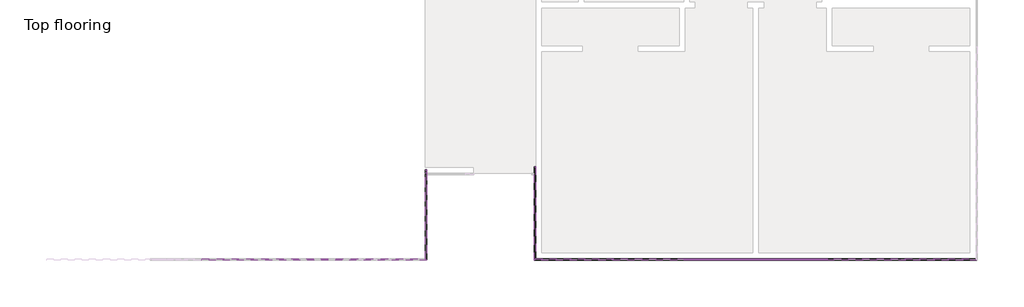
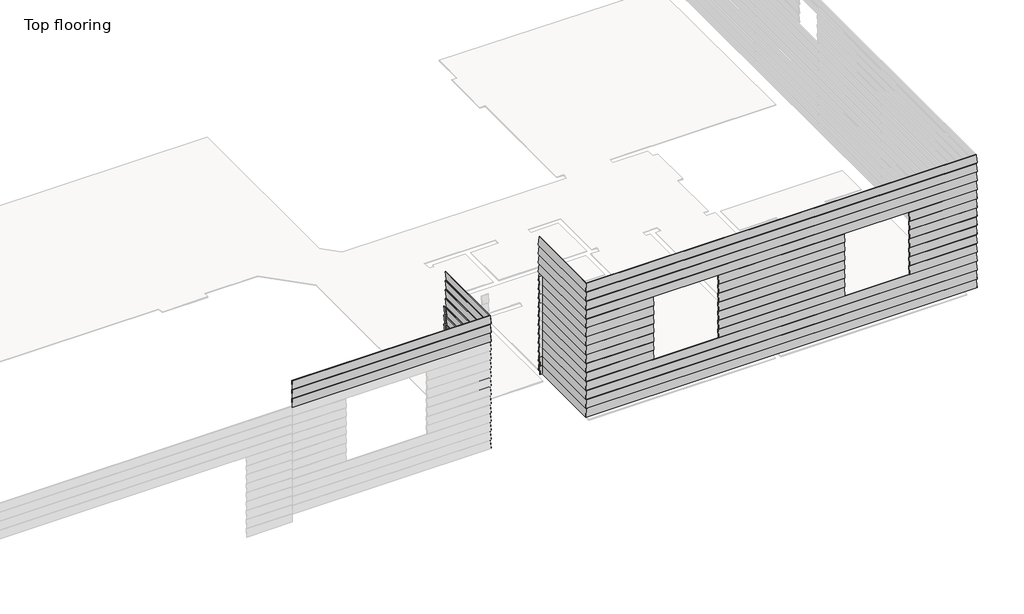
# One storey, part 2 of 5: 50 proxies.
"""IFC4 building model written with IfcOpenShell, lengths in millimetres."""

import ifcopenshell
import ifcopenshell.guid

model = None  # the IFC model being written
_history = None  # IfcOwnerHistory: only IFC2X3 demands one
_inside = {}  # id of a spatial element -> (the spatial element, [elements in it])
_under = {}  # id of a project, library or spatial element -> (it, [spatial elements below it])
_declared = {}  # id of a project -> (the project, [libraries it declares])
_typed = {}  # id of a type object -> (the type object, [elements of that type])
_made_of = {}  # id of a material, layer set ... -> (it, [elements and type objects made of it])


def new_model(schema):
    """Start an empty IFC model of exactly this schema.

    Asked for "IFC4X3", IfcOpenShell would pick the latest addendum, in which some entities
    have other attributes; the version numbers below select the first issue.
    IFC2X3 requires an IfcOwnerHistory on every rooted entity: one is made here for all.
    """
    global model, _history
    if schema == "IFC4X3":
        model = ifcopenshell.file(schema_version=(4, 3, 0, 0))
    else:
        model = ifcopenshell.file(schema=schema)
    _inside.clear()
    _under.clear()
    _declared.clear()
    _typed.clear()
    _made_of.clear()
    _history = None
    if model.schema == "IFC2X3":
        org = make("IfcOrganization", Name="unknown")
        user = make(
            "IfcPersonAndOrganization",
            ThePerson=make("IfcPerson", FamilyName="unknown"),
            TheOrganization=org,
        )
        app = make(
            "IfcApplication",
            ApplicationDeveloper=org,
            Version="unknown",
            ApplicationFullName="unknown",
            ApplicationIdentifier="unknown",
        )
        _history = make(
            "IfcOwnerHistory",
            OwningUser=user,
            OwningApplication=app,
            ChangeAction="ADDED",
            CreationDate=0,
        )
    return model


def make(cls, **values):
    """One entity of the class cls with the attributes given. An attribute that is None is left unset."""
    return model.create_entity(
        cls, **{name: value for name, value in values.items() if value is not None}
    )


def rooted(cls, **values):
    """An entity with a GlobalId (a new one), such as an element, a storey or a relation."""
    return make(cls, GlobalId=ifcopenshell.guid.new(), OwnerHistory=_history, **values)


def si_unit(unit_type, name, prefix=None):
    """IfcSIUnit, for example si_unit("LENGTHUNIT", "METRE", prefix="MILLI")."""
    return make("IfcSIUnit", UnitType=unit_type, Prefix=prefix, Name=name)


def assignment(units):
    """IfcUnitAssignment: the units of a project."""
    return None if units is None else make("IfcUnitAssignment", Units=units)


def point(xyz):
    """IfcCartesianPoint."""
    return None if xyz is None else make("IfcCartesianPoint", Coordinates=xyz)


def direction(xyz):
    """IfcDirection."""
    return None if xyz is None else make("IfcDirection", DirectionRatios=xyz)


def frame(location, z_axis=None, x_axis=None):
    """IfcAxis2Placement3D, a coordinate frame: its origin and axes. An axis left out is left unset."""
    return make(
        "IfcAxis2Placement3D",
        Location=point(location),
        Axis=direction(z_axis),
        RefDirection=direction(x_axis),
    )


def origin():
    """The frame at (0, 0, 0) with its axes left unset."""
    return frame((0.0, 0.0, 0.0))


def place(relative_to, where):
    """IfcLocalPlacement: puts the frame where relative to a parent placement (None: the world)."""
    return make(
        "IfcLocalPlacement", PlacementRelTo=relative_to, RelativePlacement=where
    )


def context(
    kind, dimensions, precision=None, world=None, true_north=None, identifier=None
):
    """IfcGeometricRepresentationContext, for example the 3D "Model" context."""
    return make(
        "IfcGeometricRepresentationContext",
        ContextIdentifier=identifier,
        ContextType=kind,
        CoordinateSpaceDimension=dimensions,
        Precision=precision,
        WorldCoordinateSystem=world,
        TrueNorth=true_north,
    )


def project(units=None, contexts=None):
    """IfcProject with its units and contexts."""
    return rooted(
        "IfcProject",
        Name="project",
        RepresentationContexts=contexts,
        UnitsInContext=assignment(units),
    )


def spatial(cls, under=None, at=None, **own):
    """A site, building, storey or space (cls), placed at a placement, below another one or the project."""
    s = rooted(cls, ObjectPlacement=at, **own)
    if under is not None:
        _under.setdefault(under.id(), (under, []))[1].append(s)
    return s


def polyline(points):
    """IfcPolyline through the points."""
    return make("IfcPolyline", Points=[point(p) for p in points])


def outline(outer, holes=None, kind="AREA"):
    """IfcArbitraryClosedProfileDef: a profile drawn as a closed curve; with holes, ...WithVoids."""
    if holes is None:
        return make("IfcArbitraryClosedProfileDef", ProfileType=kind, OuterCurve=outer)
    return make(
        "IfcArbitraryProfileDefWithVoids",
        ProfileType=kind,
        OuterCurve=outer,
        InnerCurves=holes,
    )


def extrude(swept, where, along, depth):
    """IfcExtrudedAreaSolid: the profile swept, set in the frame where, extruded along a direction by depth."""
    return make(
        "IfcExtrudedAreaSolid",
        SweptArea=swept,
        Position=where,
        ExtrudedDirection=direction(along),
        Depth=depth,
    )


def faces_of(points, faces, orient=None, outer=None):
    """IfcFace entities. A face is a list of loops; a loop is a list of indices into points, from 0.

    orient and outer hold one flag for each loop. By default every Orientation is true, the
    first loop of a face is its IfcFaceOuterBound and the others are IfcFaceBound.
    """
    made = []
    for i, loops in enumerate(faces):
        bounds = []
        for j, loop in enumerate(loops):
            is_outer = j == 0 if outer is None else outer[i][j]
            bounds.append(
                make(
                    "IfcFaceOuterBound" if is_outer else "IfcFaceBound",
                    Bound=make("IfcPolyLoop", Polygon=[points[k] for k in loop]),
                    Orientation=True if orient is None else orient[i][j],
                )
            )
        made.append(make("IfcFace", Bounds=bounds))
    return made


def faceted_brep(points, faces, orient=None, outer=None, voids=None):
    """IfcFacetedBrep: a solid bounded by flat faces; with voids (closed shells), ...WithVoids."""
    shared = [point(p) for p in points]
    hull = make("IfcClosedShell", CfsFaces=faces_of(shared, faces, orient, outer))
    if voids is None:
        return make("IfcFacetedBrep", Outer=hull)
    return make(
        "IfcFacetedBrepWithVoids",
        Outer=hull,
        Voids=[
            make(cls, CfsFaces=faces_of(shared, fs, o, b)) for cls, fs, o, b in voids
        ],
    )


def shape(context_of_items, identifier, shape_type, items):
    """IfcShapeRepresentation: the items that make up one representation, for example the "Body"."""
    return make(
        "IfcShapeRepresentation",
        ContextOfItems=context_of_items,
        RepresentationIdentifier=identifier,
        RepresentationType=shape_type,
        Items=items,
    )


def made_of(thing, what):
    """Note that an element or type object is made of a material, layer set ...; save() writes the relation."""
    if what is not None:
        _made_of.setdefault(what.id(), (what, []))[1].append(thing)
    return thing


def element(
    cls,
    number,
    at=None,
    inside=None,
    cuts=None,
    type_object=None,
    material=None,
    context=None,
    identifier="Body",
    shape_type=None,
    held_by="IfcProductDefinitionShape",
    body=None,
    shapes=None,
    **own,
):
    """One element of the class cls, such as IfcWall. Its Tag is "e" and its number.

    at: its placement. inside: the storey or other place that contains it. cuts: it is an
    opening in that element (IfcRelVoidsElement). A single representation is given by context,
    identifier, shape_type and body (its items); several are given by shapes. held_by: the class
    of the entity that holds the representations. save() writes the other relations.
    """
    e = rooted(cls, Tag="e%d" % number, ObjectPlacement=at, **own)
    if body is not None:
        shapes = [shape(context, identifier, shape_type, body)]
    if shapes is not None:
        e.Representation = make(held_by, Representations=shapes)
    if inside is not None:
        _inside.setdefault(inside.id(), (inside, []))[1].append(e)
    if cuts is not None:
        rooted(
            "IfcRelVoidsElement", RelatingBuildingElement=cuts, RelatedOpeningElement=e
        )
    if type_object is not None:
        _typed.setdefault(type_object.id(), (type_object, []))[1].append(e)
    return made_of(e, material)


def aggregate(whole, parts):
    """IfcRelAggregates: a whole, such as a stair, and the parts it consists of."""
    return rooted("IfcRelAggregates", RelatingObject=whole, RelatedObjects=parts)


def save(model, path):
    """Write the relations noted so far, then the file.

    IfcRelAggregates (storeys below a building ...), IfcRelContainedInSpatialStructure (elements
    in a storey), IfcRelDefinesByType, IfcRelAssociatesMaterial and IfcRelDeclares: one each for
    every whole, place, type object, material and project.
    """
    for whole, parts in _under.values():
        aggregate(whole, parts)
    for where, things in _inside.values():
        rooted(
            "IfcRelContainedInSpatialStructure",
            RelatedElements=things,
            RelatingStructure=where,
        )
    for kind, things in _typed.values():
        rooted("IfcRelDefinesByType", RelatedObjects=things, RelatingType=kind)
    for what, things in _made_of.values():
        rooted("IfcRelAssociatesMaterial", RelatedObjects=things, RelatingMaterial=what)
    for by, libraries in _declared.values():
        rooted("IfcRelDeclares", RelatingContext=by, RelatedDefinitions=libraries)
    model.write(path)


model = new_model("IFC4")

# Units and contexts
model_context = context("Model", 3, world=origin())
ifc_project = project(units=[si_unit("LENGTHUNIT", "METRE", prefix="MILLI")], contexts=[model_context])

# Site, building, storey
site = spatial("IfcSite", under=ifc_project)
building = spatial("IfcBuilding", under=site)
storey = spatial("IfcBuildingStorey", under=building, Name="Top flooring", Elevation=12.7)

# Proxies
placement = place(None, origin())
element("IfcBuildingElementProxy", 1, Name="Wall Sweeps", at=placement, inside=storey, context=model_context, shape_type="Brep", body=[
    faceted_brep([(-7413.8787386, -5078.007679, 179.3151454), (-7428.0541529, -5063.8322648, 338.6859634), (-7438.014829, -5053.8715886, 337.8), (-7423.8394147, -5068.0470029, 178.429182), (-7413.8787386, -3576.793764, 179.3151454), (-7423.8394147, -3576.793764, 178.429182), (-7438.014829, -3576.793764, 337.8), (-7428.0541529, -3576.793764, 338.6859634)], [[[0, 1, 2, 3]], [[4, 5, 6, 7]], [[1, 0, 4, 7]], [[2, 1, 7, 6]], [[3, 2, 6, 5]], [[0, 3, 5, 4]]]),
])
element("IfcBuildingElementProxy", 2, Name="Wall Sweeps", at=placement, inside=storey, context=model_context, shape_type="Brep", body=[
    faceted_brep([(-7413.8787386, -5078.007679, 357.1151454), (-7428.0541529, -5063.8322648, 516.4859634), (-7438.014829, -5053.8715886, 515.6), (-7423.8394147, -5068.0470029, 356.229182), (-7413.8787386, -3576.793764, 357.1151454), (-7423.8394147, -3576.793764, 356.229182), (-7438.014829, -3576.793764, 515.6), (-7428.0541529, -3576.793764, 516.4859634)], [[[0, 1, 2, 3]], [[4, 5, 6, 7]], [[1, 0, 4, 7]], [[2, 1, 7, 6]], [[3, 2, 6, 5]], [[0, 3, 5, 4]]]),
])
element("IfcBuildingElementProxy", 3, Name="Wall Sweeps", at=placement, inside=storey, context=model_context, shape_type="Brep", body=[
    faceted_brep([(-7413.8787386, -5078.007679, 534.9151454), (-7428.0541529, -5063.8322648, 694.2859634), (-7438.014829, -5053.8715886, 693.4), (-7423.8394147, -5068.0470029, 534.029182), (-7413.8787386, -3576.793764, 534.9151454), (-7423.8394147, -3576.793764, 534.029182), (-7438.014829, -3576.793764, 693.4), (-7428.0541529, -3576.793764, 694.2859634)], [[[0, 1, 2, 3]], [[4, 5, 6, 7]], [[1, 0, 4, 7]], [[2, 1, 7, 6]], [[3, 2, 6, 5]], [[0, 3, 5, 4]]]),
])
element("IfcBuildingElementProxy", 4, Name="Wall Sweeps", at=placement, inside=storey, context=model_context, shape_type="Brep", body=[
    faceted_brep([(-7413.8787386, -5078.007679, 712.7151454), (-7428.0541529, -5063.8322648, 872.0859634), (-7438.014829, -5053.8715886, 871.2), (-7423.8394147, -5068.0470029, 711.829182), (-7413.8787386, -3576.793764, 712.7151454), (-7423.8394147, -3576.793764, 711.829182), (-7438.014829, -3576.793764, 871.2), (-7428.0541529, -3576.793764, 872.0859634)], [[[0, 1, 2, 3]], [[4, 5, 6, 7]], [[1, 0, 4, 7]], [[2, 1, 7, 6]], [[3, 2, 6, 5]], [[0, 3, 5, 4]]]),
])
element("IfcBuildingElementProxy", 5, Name="Wall Sweeps", at=placement, inside=storey, context=model_context, shape_type="Brep", body=[
    faceted_brep([(-7413.8787386, -5078.007679, 890.5151454), (-7428.0541529, -5063.8322648, 1049.8859634), (-7438.014829, -5053.8715886, 1049.0), (-7423.8394147, -5068.0470029, 889.629182), (-7413.8787386, -3576.793764, 890.5151454), (-7423.8394147, -3576.793764, 889.629182), (-7438.014829, -3576.793764, 1049.0), (-7428.0541529, -3576.793764, 1049.8859634)], [[[0, 1, 2, 3]], [[4, 5, 6, 7]], [[1, 0, 4, 7]], [[2, 1, 7, 6]], [[3, 2, 6, 5]], [[0, 3, 5, 4]]]),
])
element("IfcBuildingElementProxy", 6, Name="Wall Sweeps", at=placement, inside=storey, context=model_context, shape_type="Brep", body=[
    faceted_brep([(-7413.8787386, -5078.007679, 1068.3151454), (-7428.0541529, -5063.8322648, 1227.6859634), (-7438.014829, -5053.8715886, 1226.8), (-7423.8394147, -5068.0470029, 1067.429182), (-7413.8787386, -3576.793764, 1068.3151454), (-7423.8394147, -3576.793764, 1067.429182), (-7438.014829, -3576.793764, 1226.8), (-7428.0541529, -3576.793764, 1227.6859634)], [[[0, 1, 2, 3]], [[4, 5, 6, 7]], [[1, 0, 4, 7]], [[2, 1, 7, 6]], [[3, 2, 6, 5]], [[0, 3, 5, 4]]]),
])
element("IfcBuildingElementProxy", 7, Name="Wall Sweeps", at=placement, inside=storey, context=model_context, shape_type="Brep", body=[
    faceted_brep([(-7413.8787386, -5078.007679, 1246.1151454), (-7428.0541529, -5063.8322648, 1405.4859634), (-7438.014829, -5053.8715886, 1404.6), (-7423.8394147, -5068.0470029, 1245.229182), (-7413.8787386, -3576.793764, 1246.1151454), (-7423.8394147, -3576.793764, 1245.229182), (-7438.014829, -3576.793764, 1404.6), (-7428.0541529, -3576.793764, 1405.4859634)], [[[0, 1, 2, 3]], [[4, 5, 6, 7]], [[1, 0, 4, 7]], [[2, 1, 7, 6]], [[3, 2, 6, 5]], [[0, 3, 5, 4]]]),
])
element("IfcBuildingElementProxy", 8, Name="Wall Sweeps", at=placement, inside=storey, context=model_context, shape_type="Brep", body=[
    faceted_brep([(-7413.8787386, -5078.007679, 1423.9151454), (-7428.0541529, -5063.8322648, 1583.2859634), (-7438.014829, -5053.8715886, 1582.4), (-7423.8394147, -5068.0470029, 1423.029182), (-7413.8787386, -3576.793764, 1423.9151454), (-7423.8394147, -3576.793764, 1423.029182), (-7438.014829, -3576.793764, 1582.4), (-7428.0541529, -3576.793764, 1583.2859634)], [[[0, 1, 2, 3]], [[4, 5, 6, 7]], [[1, 0, 4, 7]], [[2, 1, 7, 6]], [[3, 2, 6, 5]], [[0, 3, 5, 4]]]),
])
element("IfcBuildingElementProxy", 9, Name="Wall Sweeps", at=placement, inside=storey, context=model_context, shape_type="Brep", body=[
    faceted_brep([(-7413.8787386, -5078.007679, 1601.7151454), (-7428.0541529, -5063.8322648, 1761.0859634), (-7438.014829, -5053.8715886, 1760.2), (-7423.8394147, -5068.0470029, 1600.829182), (-7413.8787386, -3576.793764, 1601.7151454), (-7423.8394147, -3576.793764, 1600.829182), (-7438.014829, -3576.793764, 1760.2), (-7428.0541529, -3576.793764, 1761.0859634)], [[[0, 1, 2, 3]], [[4, 5, 6, 7]], [[1, 0, 4, 7]], [[2, 1, 7, 6]], [[3, 2, 6, 5]], [[0, 3, 5, 4]]]),
])
element("IfcBuildingElementProxy", 10, Name="Wall Sweeps", at=placement, inside=storey, context=model_context, shape_type="Brep", body=[
    faceted_brep([(-7413.8787386, -5078.007679, 1779.5151454), (-7428.0541529, -5063.8322648, 1938.8859634), (-7438.014829, -5053.8715886, 1938.0), (-7423.8394147, -5068.0470029, 1778.629182), (-7413.8787386, -3576.793764, 1779.5151454), (-7423.8394147, -3576.793764, 1778.629182), (-7438.014829, -3576.793764, 1938.0), (-7428.0541529, -3576.793764, 1938.8859634)], [[[0, 1, 2, 3]], [[4, 5, 6, 7]], [[1, 0, 4, 7]], [[2, 1, 7, 6]], [[3, 2, 6, 5]], [[0, 3, 5, 4]]]),
])
element("IfcBuildingElementProxy", 11, Name="Wall Sweeps", at=placement, inside=storey, context=model_context, shape_type="Brep", body=[
    faceted_brep([(-7413.8787386, -5078.007679, 1957.3151454), (-7428.0541529, -5063.8322648, 2116.6859634), (-7438.014829, -5053.8715886, 2115.8), (-7423.8394147, -5068.0470029, 1956.429182), (-7413.8787386, -3576.793764, 1957.3151454), (-7423.8394147, -3576.793764, 1956.429182), (-7438.014829, -3576.793764, 2115.8), (-7428.0541529, -3576.793764, 2116.6859634)], [[[0, 1, 2, 3]], [[4, 5, 6, 7]], [[1, 0, 4, 7]], [[2, 1, 7, 6]], [[3, 2, 6, 5]], [[0, 3, 5, 4]]]),
])
element("IfcBuildingElementProxy", 12, Name="Wall Sweeps", at=placement, inside=storey, context=model_context, shape_type="Brep", body=[
    faceted_brep([(-7413.8787386, -5078.007679, 2135.1151454), (-7428.0541529, -5063.8322648, 2294.4859634), (-7438.014829, -5053.8715886, 2293.6), (-7423.8394147, -5068.0470029, 2134.229182), (-7413.8787386, -3624.418764, 2135.1151454), (-7423.8394147, -3624.418764, 2134.229182), (-7438.014829, -3624.418764, 2293.6), (-7428.0541529, -3624.418764, 2294.4859634)], [[[0, 1, 2, 3]], [[4, 5, 6, 7]], [[1, 0, 4, 7]], [[2, 1, 7, 6]], [[3, 2, 6, 5]], [[0, 3, 5, 4]]]),
])
element("IfcBuildingElementProxy", 13, Name="Wall Sweeps", at=placement, inside=storey, context=model_context, shape_type="Brep", body=[
    faceted_brep([(-7413.8787386, -5078.007679, 2312.9151454), (-7428.0541529, -5063.8322648, 2472.2859634), (-7438.014829, -5053.8715886, 2471.4), (-7423.8394147, -5068.0470029, 2312.029182), (-7413.8787386, -3624.418764, 2312.9151454), (-7423.8394147, -3624.418764, 2312.029182), (-7438.014829, -3624.418764, 2471.4), (-7428.0541529, -3624.418764, 2472.2859634)], [[[0, 1, 2, 3]], [[4, 5, 6, 7]], [[1, 0, 4, 7]], [[2, 1, 7, 6]], [[3, 2, 6, 5]], [[0, 3, 5, 4]]]),
])
element("IfcBuildingElementProxy", 14, Name="Wall Sweeps", at=placement, inside=storey, context=model_context, shape_type="Brep", body=[
    faceted_brep([(-7413.8787386, -5078.007679, 2490.7151454), (-7428.0541529, -5063.8322648, 2650.0859634), (-7438.014829, -5053.8715886, 2649.2), (-7423.8394147, -5068.0470029, 2489.829182), (-7413.8787386, -3624.418764, 2490.7151454), (-7423.8394147, -3624.418764, 2489.829182), (-7438.014829, -3624.418764, 2649.2), (-7428.0541529, -3624.418764, 2650.0859634)], [[[0, 1, 2, 3]], [[4, 5, 6, 7]], [[1, 0, 4, 7]], [[2, 1, 7, 6]], [[3, 2, 6, 5]], [[0, 3, 5, 4]]]),
])
element("IfcBuildingElementProxy", 15, Name="Wall Sweeps", at=placement, inside=storey, context=model_context, shape_type="Brep", body=[
    faceted_brep([(-7413.8787386, -5078.007679, 2668.5151454), (-7428.0541529, -5063.8322648, 2827.8859634), (-7438.014829, -5053.8715886, 2827.0), (-7423.8394147, -5068.0470029, 2667.629182), (-7413.8787386, -3624.418764, 2668.5151454), (-7423.8394147, -3624.418764, 2667.629182), (-7438.014829, -3624.418764, 2827.0), (-7428.0541529, -3624.418764, 2827.8859634)], [[[0, 1, 2, 3]], [[4, 5, 6, 7]], [[1, 0, 4, 7]], [[2, 1, 7, 6]], [[3, 2, 6, 5]], [[0, 3, 5, 4]]]),
])
element("IfcBuildingElementProxy", 16, Name="Wall Sweeps", at=placement, inside=storey, context=model_context, shape_type="SweptSolid", body=[
    extrude(outline(polyline([(0.0, -10.0), (0.0, 0.0), (63.9, 0.0), (63.9, -10.0), (0.0, -10.0)])), frame((-5673.114829, -3645.6470029, 178.429182), z_axis=(0.0, 0.08859633935570814, 0.9960676124906221), x_axis=(1.0, 0.0, 0.0)), (0.0, 0.0, 1.0), 160.0),
    extrude(outline(polyline([(0.0, -10.0), (0.0, 0.0), (800.5, 0.0), (800.5, -10.0), (0.0, -10.0)])), frame((-7438.014829, -3645.6470029, 178.429182), z_axis=(0.0, 0.08859633935570814, 0.9960676124906221), x_axis=(1.0, 0.0, 0.0)), (0.0, 0.0, 1.0), 160.0),
])
element("IfcBuildingElementProxy", 17, Name="Wall Sweeps", at=placement, inside=storey, context=model_context, shape_type="SweptSolid", body=[
    extrude(outline(polyline([(0.0, -10.0), (0.0, 0.0), (63.9, 0.0), (63.9, -10.0), (0.0, -10.0)])), frame((-5673.114829, -3645.6470029, 356.229182), z_axis=(0.0, 0.08859633935570814, 0.9960676124906221), x_axis=(1.0, 0.0, 0.0)), (0.0, 0.0, 1.0), 160.0),
    extrude(outline(polyline([(0.0, -10.0), (0.0, 0.0), (800.5, 0.0), (800.5, -10.0), (0.0, -10.0)])), frame((-7438.014829, -3645.6470029, 356.229182), z_axis=(0.0, 0.08859633935570814, 0.9960676124906221), x_axis=(1.0, 0.0, 0.0)), (0.0, 0.0, 1.0), 160.0),
])
element("IfcBuildingElementProxy", 18, Name="Wall Sweeps", at=placement, inside=storey, context=model_context, shape_type="Brep", body=[
    faceted_brep([(-5633.3509195, -5078.007679, 179.3151454), (-5619.1755052, -5063.8322648, 338.6859634), (-5609.214829, -5053.8715886, 337.8), (-5623.3902433, -5068.0470029, 178.429182), (1730.1212614, -5078.007679, 179.3151454), (1720.1605853, -5068.0470029, 178.429182), (1705.985171, -5053.8715886, 337.8), (1715.9458471, -5063.8322648, 338.6859634)], [[[0, 1, 2, 3]], [[4, 5, 6, 7]], [[1, 0, 4, 7]], [[2, 1, 7, 6]], [[3, 2, 6, 5]], [[0, 3, 5, 4]]]),
])
element("IfcBuildingElementProxy", 19, Name="Wall Sweeps", at=placement, inside=storey, context=model_context, shape_type="Brep", body=[
    faceted_brep([(-5633.3509195, -5078.007679, 357.1151454), (-5619.1755052, -5063.8322648, 516.4859634), (-5609.214829, -5053.8715886, 515.6), (-5623.3902433, -5068.0470029, 356.229182), (1730.1212614, -5078.007679, 357.1151454), (1720.1605853, -5068.0470029, 356.229182), (1705.985171, -5053.8715886, 515.6), (1715.9458471, -5063.8322648, 516.4859634)], [[[0, 1, 2, 3]], [[4, 5, 6, 7]], [[1, 0, 4, 7]], [[2, 1, 7, 6]], [[3, 2, 6, 5]], [[0, 3, 5, 4]]]),
])
element("IfcBuildingElementProxy", 20, Name="Wall Sweeps", at=placement, inside=storey, context=model_context, shape_type="Brep", body=[
    faceted_brep([(-5633.3509195, -5078.007679, 534.9151454), (-5619.1755052, -5063.8322648, 694.2859634), (-5609.214829, -5053.8715886, 693.4), (-5623.3902433, -5068.0470029, 534.029182), (1730.1212614, -5078.007679, 534.9151454), (1720.1605853, -5068.0470029, 534.029182), (1705.985171, -5053.8715886, 693.4), (1715.9458471, -5063.8322648, 694.2859634)], [[[0, 1, 2, 3]], [[4, 5, 6, 7]], [[1, 0, 4, 7]], [[2, 1, 7, 6]], [[3, 2, 6, 5]], [[0, 3, 5, 4]]]),
])
element("IfcBuildingElementProxy", 21, Name="Wall Sweeps", at=placement, inside=storey, context=model_context, shape_type="Brep", body=[
    faceted_brep([(-5633.3509195, -5078.007679, 712.7151454), (-5619.1755052, -5063.8322648, 872.0859634), (-5609.214829, -5053.8715886, 871.2), (-5623.3902433, -5068.0470029, 711.829182), (1730.1212614, -5078.007679, 712.7151454), (1720.1605853, -5068.0470029, 711.829182), (1705.985171, -5053.8715886, 871.2), (1715.9458471, -5063.8322648, 872.0859634)], [[[0, 1, 2, 3]], [[4, 5, 6, 7]], [[1, 0, 4, 7]], [[2, 1, 7, 6]], [[3, 2, 6, 5]], [[0, 3, 5, 4]]]),
])
element("IfcBuildingElementProxy", 22, Name="Wall Sweeps", at=placement, inside=storey, context=model_context, shape_type="Brep", body=[
    faceted_brep([(455.035171, -5078.007679, 890.5151454), (455.035171, -5063.8322648, 1049.8859634), (455.035171, -5053.8715886, 1049.0), (455.035171, -5068.0470029, 889.629182), (1730.1212614, -5078.007679, 890.5151454), (1720.1605853, -5068.0470029, 889.629182), (1705.985171, -5053.8715886, 1049.0), (1715.9458471, -5063.8322648, 1049.8859634)], [[[0, 1, 2, 3]], [[4, 5, 6, 7]], [[1, 0, 4, 7]], [[2, 1, 7, 6]], [[3, 2, 6, 5]], [[0, 3, 5, 4]]]),
    faceted_brep([(-3139.064829, -5078.007679, 890.5151454), (-3139.064829, -5063.8322648, 1049.8859634), (-3139.064829, -5053.8715886, 1049.0), (-3139.064829, -5068.0470029, 889.629182), (-764.164829, -5078.007679, 890.5151454), (-764.164829, -5068.0470029, 889.629182), (-764.164829, -5053.8715886, 1049.0), (-764.164829, -5063.8322648, 1049.8859634)], [[[0, 1, 2, 3]], [[4, 5, 6, 7]], [[1, 0, 4, 7]], [[2, 1, 7, 6]], [[3, 2, 6, 5]], [[0, 3, 5, 4]]]),
    faceted_brep([(-5633.3509195, -5078.007679, 890.5151454), (-5619.1755052, -5063.8322648, 1049.8859634), (-5609.214829, -5053.8715886, 1049.0), (-5623.3902433, -5068.0470029, 889.629182), (-4358.264829, -5078.007679, 890.5151454), (-4358.264829, -5068.0470029, 889.629182), (-4358.264829, -5053.8715886, 1049.0), (-4358.264829, -5063.8322648, 1049.8859634)], [[[0, 1, 2, 3]], [[4, 5, 6, 7]], [[1, 0, 4, 7]], [[2, 1, 7, 6]], [[3, 2, 6, 5]], [[0, 3, 5, 4]]]),
])
element("IfcBuildingElementProxy", 23, Name="Wall Sweeps", at=placement, inside=storey, context=model_context, shape_type="Brep", body=[
    faceted_brep([(455.035171, -5078.007679, 1068.3151454), (455.035171, -5063.8322648, 1227.6859634), (455.035171, -5053.8715886, 1226.8), (455.035171, -5068.0470029, 1067.429182), (1730.1212614, -5078.007679, 1068.3151454), (1720.1605853, -5068.0470029, 1067.429182), (1705.985171, -5053.8715886, 1226.8), (1715.9458471, -5063.8322648, 1227.6859634)], [[[0, 1, 2, 3]], [[4, 5, 6, 7]], [[1, 0, 4, 7]], [[2, 1, 7, 6]], [[3, 2, 6, 5]], [[0, 3, 5, 4]]]),
    faceted_brep([(-3139.064829, -5078.007679, 1068.3151454), (-3139.064829, -5063.8322648, 1227.6859634), (-3139.064829, -5053.8715886, 1226.8), (-3139.064829, -5068.0470029, 1067.429182), (-764.164829, -5078.007679, 1068.3151454), (-764.164829, -5068.0470029, 1067.429182), (-764.164829, -5053.8715886, 1226.8), (-764.164829, -5063.8322648, 1227.6859634)], [[[0, 1, 2, 3]], [[4, 5, 6, 7]], [[1, 0, 4, 7]], [[2, 1, 7, 6]], [[3, 2, 6, 5]], [[0, 3, 5, 4]]]),
    faceted_brep([(-5633.3509195, -5078.007679, 1068.3151454), (-5619.1755052, -5063.8322648, 1227.6859634), (-5609.214829, -5053.8715886, 1226.8), (-5623.3902433, -5068.0470029, 1067.429182), (-4358.264829, -5078.007679, 1068.3151454), (-4358.264829, -5068.0470029, 1067.429182), (-4358.264829, -5053.8715886, 1226.8), (-4358.264829, -5063.8322648, 1227.6859634)], [[[0, 1, 2, 3]], [[4, 5, 6, 7]], [[1, 0, 4, 7]], [[2, 1, 7, 6]], [[3, 2, 6, 5]], [[0, 3, 5, 4]]]),
])
element("IfcBuildingElementProxy", 24, Name="Wall Sweeps", at=placement, inside=storey, context=model_context, shape_type="Brep", body=[
    faceted_brep([(455.035171, -5078.007679, 1246.1151454), (455.035171, -5063.8322648, 1405.4859634), (455.035171, -5053.8715886, 1404.6), (455.035171, -5068.0470029, 1245.229182), (1730.1212614, -5078.007679, 1246.1151454), (1720.1605853, -5068.0470029, 1245.229182), (1705.985171, -5053.8715886, 1404.6), (1715.9458471, -5063.8322648, 1405.4859634)], [[[0, 1, 2, 3]], [[4, 5, 6, 7]], [[1, 0, 4, 7]], [[2, 1, 7, 6]], [[3, 2, 6, 5]], [[0, 3, 5, 4]]]),
    faceted_brep([(-3139.064829, -5078.007679, 1246.1151454), (-3139.064829, -5063.8322648, 1405.4859634), (-3139.064829, -5053.8715886, 1404.6), (-3139.064829, -5068.0470029, 1245.229182), (-764.164829, -5078.007679, 1246.1151454), (-764.164829, -5068.0470029, 1245.229182), (-764.164829, -5053.8715886, 1404.6), (-764.164829, -5063.8322648, 1405.4859634)], [[[0, 1, 2, 3]], [[4, 5, 6, 7]], [[1, 0, 4, 7]], [[2, 1, 7, 6]], [[3, 2, 6, 5]], [[0, 3, 5, 4]]]),
    faceted_brep([(-5633.3509195, -5078.007679, 1246.1151454), (-5619.1755052, -5063.8322648, 1405.4859634), (-5609.214829, -5053.8715886, 1404.6), (-5623.3902433, -5068.0470029, 1245.229182), (-4358.264829, -5078.007679, 1246.1151454), (-4358.264829, -5068.0470029, 1245.229182), (-4358.264829, -5053.8715886, 1404.6), (-4358.264829, -5063.8322648, 1405.4859634)], [[[0, 1, 2, 3]], [[4, 5, 6, 7]], [[1, 0, 4, 7]], [[2, 1, 7, 6]], [[3, 2, 6, 5]], [[0, 3, 5, 4]]]),
])
element("IfcBuildingElementProxy", 25, Name="Wall Sweeps", at=placement, inside=storey, context=model_context, shape_type="Brep", body=[
    faceted_brep([(455.035171, -5078.007679, 1423.9151454), (455.035171, -5063.8322648, 1583.2859634), (455.035171, -5053.8715886, 1582.4), (455.035171, -5068.0470029, 1423.029182), (1730.1212614, -5078.007679, 1423.9151454), (1720.1605853, -5068.0470029, 1423.029182), (1705.985171, -5053.8715886, 1582.4), (1715.9458471, -5063.8322648, 1583.2859634)], [[[0, 1, 2, 3]], [[4, 5, 6, 7]], [[1, 0, 4, 7]], [[2, 1, 7, 6]], [[3, 2, 6, 5]], [[0, 3, 5, 4]]]),
    faceted_brep([(-3139.064829, -5078.007679, 1423.9151454), (-3139.064829, -5063.8322648, 1583.2859634), (-3139.064829, -5053.8715886, 1582.4), (-3139.064829, -5068.0470029, 1423.029182), (-764.164829, -5078.007679, 1423.9151454), (-764.164829, -5068.0470029, 1423.029182), (-764.164829, -5053.8715886, 1582.4), (-764.164829, -5063.8322648, 1583.2859634)], [[[0, 1, 2, 3]], [[4, 5, 6, 7]], [[1, 0, 4, 7]], [[2, 1, 7, 6]], [[3, 2, 6, 5]], [[0, 3, 5, 4]]]),
    faceted_brep([(-5633.3509195, -5078.007679, 1423.9151454), (-5619.1755052, -5063.8322648, 1583.2859634), (-5609.214829, -5053.8715886, 1582.4), (-5623.3902433, -5068.0470029, 1423.029182), (-4358.264829, -5078.007679, 1423.9151454), (-4358.264829, -5068.0470029, 1423.029182), (-4358.264829, -5053.8715886, 1582.4), (-4358.264829, -5063.8322648, 1583.2859634)], [[[0, 1, 2, 3]], [[4, 5, 6, 7]], [[1, 0, 4, 7]], [[2, 1, 7, 6]], [[3, 2, 6, 5]], [[0, 3, 5, 4]]]),
])
element("IfcBuildingElementProxy", 26, Name="Wall Sweeps", at=placement, inside=storey, context=model_context, shape_type="Brep", body=[
    faceted_brep([(455.035171, -5078.007679, 1601.7151454), (455.035171, -5063.8322648, 1761.0859634), (455.035171, -5053.8715886, 1760.2), (455.035171, -5068.0470029, 1600.829182), (1730.1212614, -5078.007679, 1601.7151454), (1720.1605853, -5068.0470029, 1600.829182), (1705.985171, -5053.8715886, 1760.2), (1715.9458471, -5063.8322648, 1761.0859634)], [[[0, 1, 2, 3]], [[4, 5, 6, 7]], [[1, 0, 4, 7]], [[2, 1, 7, 6]], [[3, 2, 6, 5]], [[0, 3, 5, 4]]]),
    faceted_brep([(-3139.064829, -5078.007679, 1601.7151454), (-3139.064829, -5063.8322648, 1761.0859634), (-3139.064829, -5053.8715886, 1760.2), (-3139.064829, -5068.0470029, 1600.829182), (-764.164829, -5078.007679, 1601.7151454), (-764.164829, -5068.0470029, 1600.829182), (-764.164829, -5053.8715886, 1760.2), (-764.164829, -5063.8322648, 1761.0859634)], [[[0, 1, 2, 3]], [[4, 5, 6, 7]], [[1, 0, 4, 7]], [[2, 1, 7, 6]], [[3, 2, 6, 5]], [[0, 3, 5, 4]]]),
    faceted_brep([(-5633.3509195, -5078.007679, 1601.7151454), (-5619.1755052, -5063.8322648, 1761.0859634), (-5609.214829, -5053.8715886, 1760.2), (-5623.3902433, -5068.0470029, 1600.829182), (-4358.264829, -5078.007679, 1601.7151454), (-4358.264829, -5068.0470029, 1600.829182), (-4358.264829, -5053.8715886, 1760.2), (-4358.264829, -5063.8322648, 1761.0859634)], [[[0, 1, 2, 3]], [[4, 5, 6, 7]], [[1, 0, 4, 7]], [[2, 1, 7, 6]], [[3, 2, 6, 5]], [[0, 3, 5, 4]]]),
])
element("IfcBuildingElementProxy", 27, Name="Wall Sweeps", at=placement, inside=storey, context=model_context, shape_type="Brep", body=[
    faceted_brep([(455.035171, -5078.007679, 1779.5151454), (455.035171, -5063.8322648, 1938.8859634), (455.035171, -5053.8715886, 1938.0), (455.035171, -5068.0470029, 1778.629182), (1730.1212614, -5078.007679, 1779.5151454), (1720.1605853, -5068.0470029, 1778.629182), (1705.985171, -5053.8715886, 1938.0), (1715.9458471, -5063.8322648, 1938.8859634)], [[[0, 1, 2, 3]], [[4, 5, 6, 7]], [[1, 0, 4, 7]], [[2, 1, 7, 6]], [[3, 2, 6, 5]], [[0, 3, 5, 4]]]),
    faceted_brep([(-3139.064829, -5078.007679, 1779.5151454), (-3139.064829, -5063.8322648, 1938.8859634), (-3139.064829, -5053.8715886, 1938.0), (-3139.064829, -5068.0470029, 1778.629182), (-764.164829, -5078.007679, 1779.5151454), (-764.164829, -5068.0470029, 1778.629182), (-764.164829, -5053.8715886, 1938.0), (-764.164829, -5063.8322648, 1938.8859634)], [[[0, 1, 2, 3]], [[4, 5, 6, 7]], [[1, 0, 4, 7]], [[2, 1, 7, 6]], [[3, 2, 6, 5]], [[0, 3, 5, 4]]]),
    faceted_brep([(-5633.3509195, -5078.007679, 1779.5151454), (-5619.1755052, -5063.8322648, 1938.8859634), (-5609.214829, -5053.8715886, 1938.0), (-5623.3902433, -5068.0470029, 1778.629182), (-4358.264829, -5078.007679, 1779.5151454), (-4358.264829, -5068.0470029, 1778.629182), (-4358.264829, -5053.8715886, 1938.0), (-4358.264829, -5063.8322648, 1938.8859634)], [[[0, 1, 2, 3]], [[4, 5, 6, 7]], [[1, 0, 4, 7]], [[2, 1, 7, 6]], [[3, 2, 6, 5]], [[0, 3, 5, 4]]]),
])
element("IfcBuildingElementProxy", 28, Name="Wall Sweeps", at=placement, inside=storey, context=model_context, shape_type="Brep", body=[
    faceted_brep([(455.035171, -5078.007679, 1957.3151454), (455.035171, -5063.8322648, 2116.6859634), (455.035171, -5053.8715886, 2115.8), (455.035171, -5068.0470029, 1956.429182), (1730.1212614, -5078.007679, 1957.3151454), (1720.1605853, -5068.0470029, 1956.429182), (1705.985171, -5053.8715886, 2115.8), (1715.9458471, -5063.8322648, 2116.6859634)], [[[0, 1, 2, 3]], [[4, 5, 6, 7]], [[1, 0, 4, 7]], [[2, 1, 7, 6]], [[3, 2, 6, 5]], [[0, 3, 5, 4]]]),
    faceted_brep([(-3139.064829, -5078.007679, 1957.3151454), (-3139.064829, -5063.8322648, 2116.6859634), (-3139.064829, -5053.8715886, 2115.8), (-3139.064829, -5068.0470029, 1956.429182), (-764.164829, -5078.007679, 1957.3151454), (-764.164829, -5068.0470029, 1956.429182), (-764.164829, -5053.8715886, 2115.8), (-764.164829, -5063.8322648, 2116.6859634)], [[[0, 1, 2, 3]], [[4, 5, 6, 7]], [[1, 0, 4, 7]], [[2, 1, 7, 6]], [[3, 2, 6, 5]], [[0, 3, 5, 4]]]),
    faceted_brep([(-5633.3509195, -5078.007679, 1957.3151454), (-5619.1755052, -5063.8322648, 2116.6859634), (-5609.214829, -5053.8715886, 2115.8), (-5623.3902433, -5068.0470029, 1956.429182), (-4358.264829, -5078.007679, 1957.3151454), (-4358.264829, -5068.0470029, 1956.429182), (-4358.264829, -5053.8715886, 2115.8), (-4358.264829, -5063.8322648, 2116.6859634)], [[[0, 1, 2, 3]], [[4, 5, 6, 7]], [[1, 0, 4, 7]], [[2, 1, 7, 6]], [[3, 2, 6, 5]], [[0, 3, 5, 4]]]),
])
element("IfcBuildingElementProxy", 29, Name="Wall Sweeps", at=placement, inside=storey, context=model_context, shape_type="Brep", body=[
    faceted_brep([(-5633.3509195, -5078.007679, 2135.1151454), (-5619.1755052, -5063.8322648, 2294.4859634), (-5609.214829, -5053.8715886, 2293.6), (-5623.3902433, -5068.0470029, 2134.229182), (1730.1212614, -5078.007679, 2135.1151454), (1720.1605853, -5068.0470029, 2134.229182), (1705.985171, -5053.8715886, 2293.6), (1715.9458471, -5063.8322648, 2294.4859634)], [[[0, 1, 2, 3]], [[4, 5, 6, 7]], [[1, 0, 4, 7]], [[2, 1, 7, 6]], [[3, 2, 6, 5]], [[0, 3, 5, 4]]]),
])
element("IfcBuildingElementProxy", 30, Name="Wall Sweeps", at=placement, inside=storey, context=model_context, shape_type="Brep", body=[
    faceted_brep([(-5633.3509195, -5078.007679, 2312.9151454), (-5619.1755052, -5063.8322648, 2472.2859634), (-5609.214829, -5053.8715886, 2471.4), (-5623.3902433, -5068.0470029, 2312.029182), (1730.1212614, -5078.007679, 2312.9151454), (1720.1605853, -5068.0470029, 2312.029182), (1705.985171, -5053.8715886, 2471.4), (1715.9458471, -5063.8322648, 2472.2859634)], [[[0, 1, 2, 3]], [[4, 5, 6, 7]], [[1, 0, 4, 7]], [[2, 1, 7, 6]], [[3, 2, 6, 5]], [[0, 3, 5, 4]]]),
])
element("IfcBuildingElementProxy", 31, Name="Wall Sweeps", at=placement, inside=storey, context=model_context, shape_type="Brep", body=[
    faceted_brep([(-5633.3509195, -5078.007679, 2490.7151454), (-5619.1755052, -5063.8322648, 2650.0859634), (-5609.214829, -5053.8715886, 2649.2), (-5623.3902433, -5068.0470029, 2489.829182), (1730.1212614, -5078.007679, 2490.7151454), (1720.1605853, -5068.0470029, 2489.829182), (1705.985171, -5053.8715886, 2649.2), (1715.9458471, -5063.8322648, 2650.0859634)], [[[0, 1, 2, 3]], [[4, 5, 6, 7]], [[1, 0, 4, 7]], [[2, 1, 7, 6]], [[3, 2, 6, 5]], [[0, 3, 5, 4]]]),
])
element("IfcBuildingElementProxy", 32, Name="Wall Sweeps", at=placement, inside=storey, context=model_context, shape_type="Brep", body=[
    faceted_brep([(-5633.3509195, -5078.007679, 2668.5151454), (-5619.1755052, -5063.8322648, 2827.8859634), (-5609.214829, -5053.8715886, 2827.0), (-5623.3902433, -5068.0470029, 2667.629182), (1730.1212614, -5078.007679, 2668.5151454), (1720.1605853, -5068.0470029, 2667.629182), (1705.985171, -5053.8715886, 2827.0), (1715.9458471, -5063.8322648, 2827.8859634)], [[[0, 1, 2, 3]], [[4, 5, 6, 7]], [[1, 0, 4, 7]], [[2, 1, 7, 6]], [[3, 2, 6, 5]], [[0, 3, 5, 4]]]),
])
element("IfcBuildingElementProxy", 33, Name="Wall Sweeps", at=placement, inside=storey, context=model_context, shape_type="Brep", body=[
    faceted_brep([(-11152.764829, -5078.007679, 2312.9151454), (-11152.764829, -5063.8322648, 2472.2859634), (-11152.764829, -5053.8715886, 2471.4), (-11152.764829, -5068.0470029, 2312.029182), (-7413.8787386, -5078.007679, 2312.9151454), (-7423.8394147, -5068.0470029, 2312.029182), (-7438.014829, -5053.8715886, 2471.4), (-7428.0541529, -5063.8322648, 2472.2859634)], [[[0, 1, 2, 3]], [[4, 5, 6, 7]], [[1, 0, 4, 7]], [[2, 1, 7, 6]], [[3, 2, 6, 5]], [[0, 3, 5, 4]]]),
])
element("IfcBuildingElementProxy", 34, Name="Wall Sweeps", at=placement, inside=storey, context=model_context, shape_type="Brep", body=[
    faceted_brep([(-11152.764829, -5078.007679, 2490.7151454), (-11152.764829, -5063.8322648, 2650.0859634), (-11152.764829, -5053.8715886, 2649.2), (-11152.764829, -5068.0470029, 2489.829182), (-7413.8787386, -5078.007679, 2490.7151454), (-7423.8394147, -5068.0470029, 2489.829182), (-7438.014829, -5053.8715886, 2649.2), (-7428.0541529, -5063.8322648, 2650.0859634)], [[[0, 1, 2, 3]], [[4, 5, 6, 7]], [[1, 0, 4, 7]], [[2, 1, 7, 6]], [[3, 2, 6, 5]], [[0, 3, 5, 4]]]),
])
element("IfcBuildingElementProxy", 35, Name="Wall Sweeps", at=placement, inside=storey, context=model_context, shape_type="Brep", body=[
    faceted_brep([(-11152.764829, -5078.007679, 2668.5151454), (-11152.764829, -5063.8322648, 2827.8859634), (-11152.764829, -5053.8715886, 2827.0), (-11152.764829, -5068.0470029, 2667.629182), (-7413.8787386, -5078.007679, 2668.5151454), (-7423.8394147, -5068.0470029, 2667.629182), (-7438.014829, -5053.8715886, 2827.0), (-7428.0541529, -5063.8322648, 2827.8859634)], [[[0, 1, 2, 3]], [[4, 5, 6, 7]], [[1, 0, 4, 7]], [[2, 1, 7, 6]], [[3, 2, 6, 5]], [[0, 3, 5, 4]]]),
])
element("IfcBuildingElementProxy", 36, Name="Wall Sweeps", at=placement, inside=storey, context=model_context, shape_type="Brep", body=[
    faceted_brep([(-5633.3509195, -5078.007679, 179.3151454), (-5623.3902433, -5068.0470029, 178.429182), (-5609.214829, -5053.8715886, 337.8), (-5619.1755052, -5063.8322648, 338.6859634), (-5633.3509195, -3528.3810879, 179.3151454), (-5619.1755052, -3528.3810879, 338.6859634), (-5609.214829, -3528.3810879, 337.8), (-5623.3902433, -3528.3810879, 178.429182)], [[[0, 1, 2, 3]], [[4, 5, 6, 7]], [[1, 0, 4, 7]], [[2, 1, 7, 6]], [[3, 2, 6, 5]], [[0, 3, 5, 4]]]),
])
element("IfcBuildingElementProxy", 37, Name="Wall Sweeps", at=placement, inside=storey, context=model_context, shape_type="Brep", body=[
    faceted_brep([(-5633.3509195, -5078.007679, 357.1151454), (-5623.3902433, -5068.0470029, 356.229182), (-5609.214829, -5053.8715886, 515.6), (-5619.1755052, -5063.8322648, 516.4859634), (-5633.3509195, -3528.3810879, 357.1151454), (-5619.1755052, -3528.3810879, 516.4859634), (-5609.214829, -3528.3810879, 515.6), (-5623.3902433, -3528.3810879, 356.229182)], [[[0, 1, 2, 3]], [[4, 5, 6, 7]], [[1, 0, 4, 7]], [[2, 1, 7, 6]], [[3, 2, 6, 5]], [[0, 3, 5, 4]]]),
])
element("IfcBuildingElementProxy", 38, Name="Wall Sweeps", at=placement, inside=storey, context=model_context, shape_type="Brep", body=[
    faceted_brep([(-5633.3509195, -5078.007679, 534.9151454), (-5623.3902433, -5068.0470029, 534.029182), (-5609.214829, -5053.8715886, 693.4), (-5619.1755052, -5063.8322648, 694.2859634), (-5633.3509195, -3528.3810879, 534.9151454), (-5619.1755052, -3528.3810879, 694.2859634), (-5609.214829, -3528.3810879, 693.4), (-5623.3902433, -3528.3810879, 534.029182)], [[[0, 1, 2, 3]], [[4, 5, 6, 7]], [[1, 0, 4, 7]], [[2, 1, 7, 6]], [[3, 2, 6, 5]], [[0, 3, 5, 4]]]),
])
element("IfcBuildingElementProxy", 39, Name="Wall Sweeps", at=placement, inside=storey, context=model_context, shape_type="Brep", body=[
    faceted_brep([(-5633.3509195, -5078.007679, 712.7151454), (-5623.3902433, -5068.0470029, 711.829182), (-5609.214829, -5053.8715886, 871.2), (-5619.1755052, -5063.8322648, 872.0859634), (-5633.3509195, -3528.3810879, 712.7151454), (-5619.1755052, -3528.3810879, 872.0859634), (-5609.214829, -3528.3810879, 871.2), (-5623.3902433, -3528.3810879, 711.829182)], [[[0, 1, 2, 3]], [[4, 5, 6, 7]], [[1, 0, 4, 7]], [[2, 1, 7, 6]], [[3, 2, 6, 5]], [[0, 3, 5, 4]]]),
])
element("IfcBuildingElementProxy", 40, Name="Wall Sweeps", at=placement, inside=storey, context=model_context, shape_type="Brep", body=[
    faceted_brep([(-5633.3509195, -5078.007679, 890.5151454), (-5623.3902433, -5068.0470029, 889.629182), (-5609.214829, -5053.8715886, 1049.0), (-5619.1755052, -5063.8322648, 1049.8859634), (-5633.3509195, -3528.3810879, 890.5151454), (-5619.1755052, -3528.3810879, 1049.8859634), (-5609.214829, -3528.3810879, 1049.0), (-5623.3902433, -3528.3810879, 889.629182)], [[[0, 1, 2, 3]], [[4, 5, 6, 7]], [[1, 0, 4, 7]], [[2, 1, 7, 6]], [[3, 2, 6, 5]], [[0, 3, 5, 4]]]),
])
element("IfcBuildingElementProxy", 41, Name="Wall Sweeps", at=placement, inside=storey, context=model_context, shape_type="Brep", body=[
    faceted_brep([(-5633.3509195, -5078.007679, 1068.3151454), (-5623.3902433, -5068.0470029, 1067.429182), (-5609.214829, -5053.8715886, 1226.8), (-5619.1755052, -5063.8322648, 1227.6859634), (-5633.3509195, -3528.3810879, 1068.3151454), (-5619.1755052, -3528.3810879, 1227.6859634), (-5609.214829, -3528.3810879, 1226.8), (-5623.3902433, -3528.3810879, 1067.429182)], [[[0, 1, 2, 3]], [[4, 5, 6, 7]], [[1, 0, 4, 7]], [[2, 1, 7, 6]], [[3, 2, 6, 5]], [[0, 3, 5, 4]]]),
])
element("IfcBuildingElementProxy", 42, Name="Wall Sweeps", at=placement, inside=storey, context=model_context, shape_type="Brep", body=[
    faceted_brep([(-5633.3509195, -5078.007679, 1246.1151454), (-5623.3902433, -5068.0470029, 1245.229182), (-5609.214829, -5053.8715886, 1404.6), (-5619.1755052, -5063.8322648, 1405.4859634), (-5633.3509195, -3528.3810879, 1246.1151454), (-5619.1755052, -3528.3810879, 1405.4859634), (-5609.214829, -3528.3810879, 1404.6), (-5623.3902433, -3528.3810879, 1245.229182)], [[[0, 1, 2, 3]], [[4, 5, 6, 7]], [[1, 0, 4, 7]], [[2, 1, 7, 6]], [[3, 2, 6, 5]], [[0, 3, 5, 4]]]),
])
element("IfcBuildingElementProxy", 43, Name="Wall Sweeps", at=placement, inside=storey, context=model_context, shape_type="Brep", body=[
    faceted_brep([(-5633.3509195, -5078.007679, 1423.9151454), (-5623.3902433, -5068.0470029, 1423.029182), (-5609.214829, -5053.8715886, 1582.4), (-5619.1755052, -5063.8322648, 1583.2859634), (-5633.3509195, -3528.3810879, 1423.9151454), (-5619.1755052, -3528.3810879, 1583.2859634), (-5609.214829, -3528.3810879, 1582.4), (-5623.3902433, -3528.3810879, 1423.029182)], [[[0, 1, 2, 3]], [[4, 5, 6, 7]], [[1, 0, 4, 7]], [[2, 1, 7, 6]], [[3, 2, 6, 5]], [[0, 3, 5, 4]]]),
])
element("IfcBuildingElementProxy", 44, Name="Wall Sweeps", at=placement, inside=storey, context=model_context, shape_type="Brep", body=[
    faceted_brep([(-5633.3509195, -5078.007679, 1601.7151454), (-5623.3902433, -5068.0470029, 1600.829182), (-5609.214829, -5053.8715886, 1760.2), (-5619.1755052, -5063.8322648, 1761.0859634), (-5633.3509195, -3528.3810879, 1601.7151454), (-5619.1755052, -3528.3810879, 1761.0859634), (-5609.214829, -3528.3810879, 1760.2), (-5623.3902433, -3528.3810879, 1600.829182)], [[[0, 1, 2, 3]], [[4, 5, 6, 7]], [[1, 0, 4, 7]], [[2, 1, 7, 6]], [[3, 2, 6, 5]], [[0, 3, 5, 4]]]),
])
element("IfcBuildingElementProxy", 45, Name="Wall Sweeps", at=placement, inside=storey, context=model_context, shape_type="Brep", body=[
    faceted_brep([(-5633.3509195, -5078.007679, 1779.5151454), (-5623.3902433, -5068.0470029, 1778.629182), (-5609.214829, -5053.8715886, 1938.0), (-5619.1755052, -5063.8322648, 1938.8859634), (-5633.3509195, -3528.3810879, 1779.5151454), (-5619.1755052, -3528.3810879, 1938.8859634), (-5609.214829, -3528.3810879, 1938.0), (-5623.3902433, -3528.3810879, 1778.629182)], [[[0, 1, 2, 3]], [[4, 5, 6, 7]], [[1, 0, 4, 7]], [[2, 1, 7, 6]], [[3, 2, 6, 5]], [[0, 3, 5, 4]]]),
])
element("IfcBuildingElementProxy", 46, Name="Wall Sweeps", at=placement, inside=storey, context=model_context, shape_type="Brep", body=[
    faceted_brep([(-5633.3509195, -5078.007679, 1957.3151454), (-5623.3902433, -5068.0470029, 1956.429182), (-5609.214829, -5053.8715886, 2115.8), (-5619.1755052, -5063.8322648, 2116.6859634), (-5633.3509195, -3528.3810879, 1957.3151454), (-5619.1755052, -3528.3810879, 2116.6859634), (-5609.214829, -3528.3810879, 2115.8), (-5623.3902433, -3528.3810879, 1956.429182)], [[[0, 1, 2, 3]], [[4, 5, 6, 7]], [[1, 0, 4, 7]], [[2, 1, 7, 6]], [[3, 2, 6, 5]], [[0, 3, 5, 4]]]),
])
element("IfcBuildingElementProxy", 47, Name="Wall Sweeps", at=placement, inside=storey, context=model_context, shape_type="Brep", body=[
    faceted_brep([(-5633.3509195, -5078.007679, 2135.1151454), (-5623.3902433, -5068.0470029, 2134.229182), (-5609.214829, -5053.8715886, 2293.6), (-5619.1755052, -5063.8322648, 2294.4859634), (-5633.3509195, -3528.3810879, 2135.1151454), (-5619.1755052, -3528.3810879, 2294.4859634), (-5609.214829, -3528.3810879, 2293.6), (-5623.3902433, -3528.3810879, 2134.229182)], [[[0, 1, 2, 3]], [[4, 5, 6, 7]], [[1, 0, 4, 7]], [[2, 1, 7, 6]], [[3, 2, 6, 5]], [[0, 3, 5, 4]]]),
])
element("IfcBuildingElementProxy", 48, Name="Wall Sweeps", at=placement, inside=storey, context=model_context, shape_type="Brep", body=[
    faceted_brep([(-5633.3509195, -5078.007679, 2312.9151454), (-5623.3902433, -5068.0470029, 2312.029182), (-5609.214829, -5053.8715886, 2471.4), (-5619.1755052, -5063.8322648, 2472.2859634), (-5633.3509195, -3528.3810879, 2312.9151454), (-5619.1755052, -3528.3810879, 2472.2859634), (-5609.214829, -3528.3810879, 2471.4), (-5623.3902433, -3528.3810879, 2312.029182)], [[[0, 1, 2, 3]], [[4, 5, 6, 7]], [[1, 0, 4, 7]], [[2, 1, 7, 6]], [[3, 2, 6, 5]], [[0, 3, 5, 4]]]),
])
element("IfcBuildingElementProxy", 49, Name="Wall Sweeps", at=placement, inside=storey, context=model_context, shape_type="Brep", body=[
    faceted_brep([(-5633.3509195, -5078.007679, 2490.7151454), (-5623.3902433, -5068.0470029, 2489.829182), (-5609.214829, -5053.8715886, 2649.2), (-5619.1755052, -5063.8322648, 2650.0859634), (-5633.3509195, -3528.3810879, 2490.7151454), (-5619.1755052, -3528.3810879, 2650.0859634), (-5609.214829, -3528.3810879, 2649.2), (-5623.3902433, -3528.3810879, 2489.829182)], [[[0, 1, 2, 3]], [[4, 5, 6, 7]], [[1, 0, 4, 7]], [[2, 1, 7, 6]], [[3, 2, 6, 5]], [[0, 3, 5, 4]]]),
])
element("IfcBuildingElementProxy", 50, Name="Wall Sweeps", at=placement, inside=storey, context=model_context, shape_type="Brep", body=[
    faceted_brep([(-5633.3509195, -5078.007679, 2668.5151454), (-5623.3902433, -5068.0470029, 2667.629182), (-5609.214829, -5053.8715886, 2827.0), (-5619.1755052, -5063.8322648, 2827.8859634), (-5633.3509195, -3528.3810879, 2668.5151454), (-5619.1755052, -3528.3810879, 2827.8859634), (-5609.214829, -3528.3810879, 2827.0), (-5623.3902433, -3528.3810879, 2667.629182)], [[[0, 1, 2, 3]], [[4, 5, 6, 7]], [[1, 0, 4, 7]], [[2, 1, 7, 6]], [[3, 2, 6, 5]], [[0, 3, 5, 4]]]),
])

save(model, "model.ifc")

# Revit data of these elements
# Project information
#   Project Issue Date = "Issue Date"
#   Project Status = "Project Status"
#   Client Name = "Owner"
#   Project Address = "Enter address here"
#   Project Name = "Project Name"
#   Project Number = "Project Number"
# Grids (mm)
#   "D": line (5817.21, -3529.872) -> (-20839.361, -3529.872)
#   "6": line (-2561.215, -7229.778) -> (-2561.215, 8272.214)
#   "4": line (-6828.415, -7229.778) -> (-6828.415, 8272.214)
#   "10": line (5817.21, -5155.472) -> (-20839.361, -5155.472)
#   "11": line (-16886.815, -7229.778) -> (-16886.815, 8272.214)
#   "14": line (-14448.415, -3894.183) -> (-14448.415, -5768.247)
#   "1": line (-17801.215, -7229.778) -> (-17801.215, 8272.214)
#   "2": line (-11152.765, -7229.778) -> (-11152.765, 8272.214)
#   "3": line (-7438.015, -7229.778) -> (-7438.015, 8272.214)
#   "5": line (-5609.215, -7229.778) -> (-5609.215, 8272.214)
#   "7": line (-1951.615, -7229.778) -> (-1951.615, 8272.214)
#   "8": line (1705.985, -7229.778) -> (1705.985, 8272.214)
#   "E": line (5817.21, -5053.872) -> (-20839.361, -5053.872)
#   "B": line (5817.21, 1226.278) -> (-20839.361, 1226.278)
#   "A": line (5817.21, 5207.728) -> (-20839.361, 5207.728)
#   "C": line (5817.21, -837.472) -> (-20839.361, -837.472)
# Elements 1, 2, 3, 4, 5, 6, 7, 8, 9, 10, 11, 12, 13, 14, 15, 16, 17, 18, 19, 20, 21, 22, 23, 24, 25, 26, 27, 28, 29, 30, 31, 32, 33, 34, 35, 36, 37, 38, 39, 40, 41, 42, 43, 44, 45, 46, 47, 48, 49, 50 (IfcBuildingElementProxy)
#   Phase Created = New Construction
#   Materials on its faces: "Aluminum"
# Materials
#   "Aluminum": class "Metal", colour RGB 244 244 244, transparency 0, Description = "Aluminum 6061", Cost = 0
